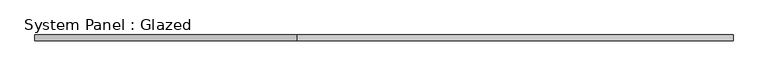
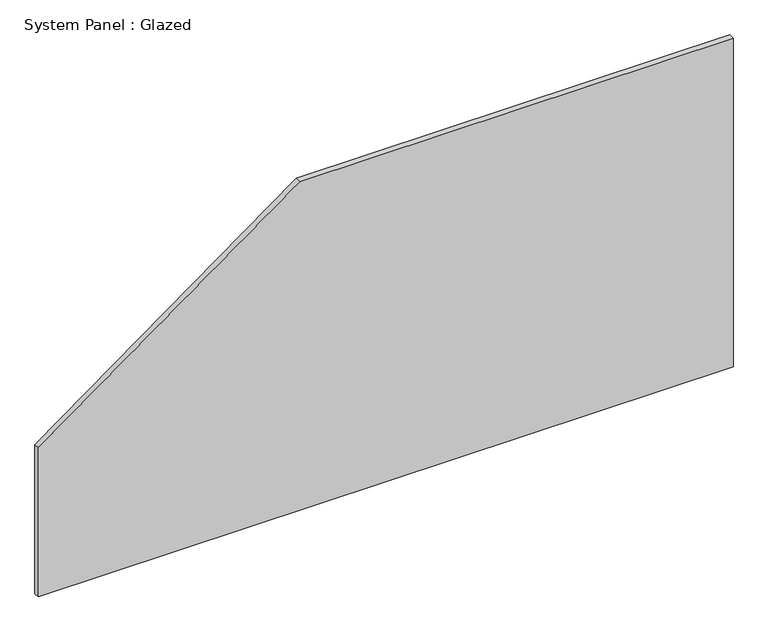
"""IFC4 building model written with IfcOpenShell, lengths in millimetres: plate geometry, System Panel : Glazed."""

from ifc_helpers import new_model, si_unit, frame, origin, place, context, project, spatial, polyline, outline, extrude, source, transform, mapped, element, save


def system_panel_glazed_6e331606(model_context):
    return source(origin(), model_context, "Body", "SweptSolid", [
        extrude(outline(polyline([(0.0, -1500.0), (0.0, 1500.0), (1500.0, 1500.0), (1500.0, -372.0214972), (680.2439122, -1500.0), (0.0, -1500.0)])), frame((0.0, 24.5, 0.0), z_axis=(0.0, 1.0, 0.0), x_axis=(0.0, 0.0, 1.0)), (0.0, 0.0, 1.0), 25.0),
    ])


if __name__ == "__main__":
    model = new_model("IFC4")
    model_context = context("Model", 3, world=origin())
    ifc_project = project(units=[si_unit("LENGTHUNIT", "METRE", prefix="MILLI")], contexts=[model_context])
    site = spatial("IfcSite", under=ifc_project)
    building = spatial("IfcBuilding", under=site)
    placement = place(None, origin())
    system_panel_glazed_shape = system_panel_glazed_6e331606(model_context)
    element("IfcPlate", 1, ObjectType="System Panel : Glazed", at=placement, inside=building, context=model_context, shape_type="MappedRepresentation", body=[
        mapped(system_panel_glazed_shape, transform((0.0, 0.0, 0.0), x_axis=(1.0, 0.0, 0.0), y_axis=(0.0, 1.0, 0.0), z_axis=(0.0, 0.0, 1.0))),
    ])
    save(model, "model.ifc")

# Revit data of these elements
# Type "System Panel : Glazed"
#   Construction Type Id = "GSP4R"
#   Analytic Construction = "1/8 in Pilkington single glazing"
#   Visual Light Transmittance = 0.9
#   Solar Heat Gain Coefficient = 0.86
#   Heat Transfer Coefficient (U) = 6.7069 W/(m²·K)
#   Define Thermal Properties by = 1
# Element 1 (IfcPlate, "System Panel : Glazed")
#   Materials on its faces: "Glass"
# Materials
#   "Glass": class "Glass", colour RGB 0 128 192, transparency 0.9, Description = "Soda Lime Glass", Cost = 0
